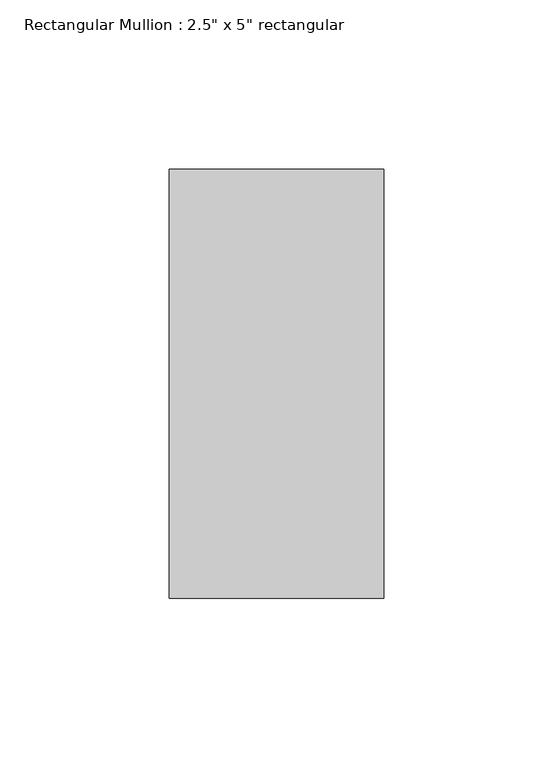
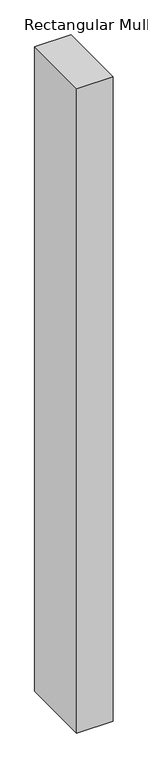
"""IFC4 building model written with IfcOpenShell, lengths in millimetres: member geometry."""

from ifc_helpers import new_model, si_unit, frame, origin, place, context, project, spatial, polyline, outline, extrude, source, transform, mapped, element, save


def member_2c3f20f2(model_context):
    return source(origin(), model_context, "Body", "SweptSolid", [
        extrude(outline(polyline([(31.75, 63.5), (31.75, -63.5), (-31.75, -63.5), (-31.75, 63.5), (31.75, 63.5)])), frame((0.0, 0.0, -1188.8151287), z_axis=(0.0, 0.0, 1.0), x_axis=(1.0, 0.0, 0.0)), (0.0, 0.0, 1.0), 1188.8151287),
    ])


if __name__ == "__main__":
    model = new_model("IFC4")
    model_context = context("Model", 3, world=origin())
    ifc_project = project(units=[si_unit("LENGTHUNIT", "METRE", prefix="MILLI")], contexts=[model_context])
    site = spatial("IfcSite", under=ifc_project)
    building = spatial("IfcBuilding", under=site)
    placement = place(None, origin())
    member_shape = member_2c3f20f2(model_context)
    element("IfcMember", 1, ObjectType="Rectangular Mullion : 2.5\" x 5\" rectangular", at=placement, inside=building, context=model_context, shape_type="MappedRepresentation", body=[
        mapped(member_shape, transform((0.0, 0.0, 0.0), x_axis=(1.0, 0.0, 0.0), y_axis=(0.0, 1.0, 0.0), z_axis=(0.0, 0.0, 1.0))),
    ])
    save(model, "model.ifc")

# Revit data of these elements
# Type "Rectangular Mullion : 2.5\" x 5\" rectangular"
#   built-in parameter 1007304 = 0.416667 (stored number, unit not read)
#   built-in parameter 1007301 = 0.104167 (stored number, unit not read)
#   built-in parameter 1007300 = 0.104167 (stored number, unit not read)
# Element 1 (IfcMember, "Rectangular Mullion : 2.5\" x 5\" rectangular")
#   Materials on its faces: "Metal - Aluminum"
# Materials
#   "Metal - Aluminum": class "Metal", colour RGB 140 140 140, transparency 0
